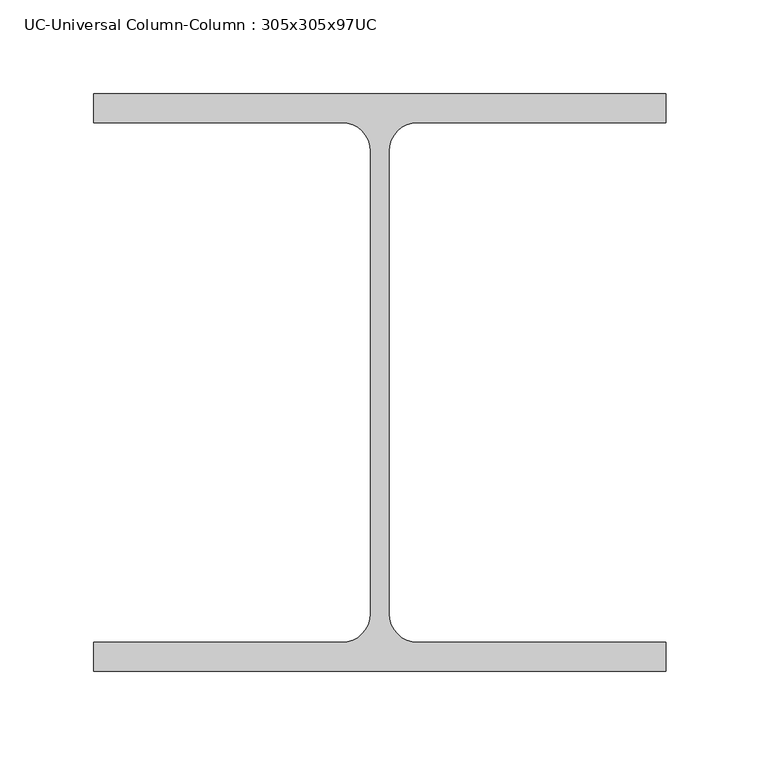
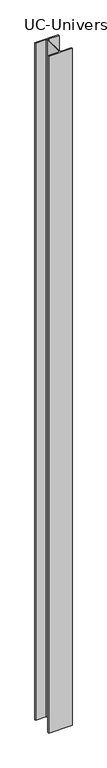
"""IFC4 building model written with IfcOpenShell, lengths in millimetres: column geometry, UC-Universal Column-Column : 305x305x97UC."""

import ifcopenshell
import ifcopenshell.guid

model = None  # the IFC model being written
_history = None  # IfcOwnerHistory: only IFC2X3 demands one
_inside = {}  # id of a spatial element -> (the spatial element, [elements in it])
_under = {}  # id of a project, library or spatial element -> (it, [spatial elements below it])
_declared = {}  # id of a project -> (the project, [libraries it declares])
_typed = {}  # id of a type object -> (the type object, [elements of that type])
_made_of = {}  # id of a material, layer set ... -> (it, [elements and type objects made of it])


def new_model(schema):
    """Start an empty IFC model of exactly this schema.

    Asked for "IFC4X3", IfcOpenShell would pick the latest addendum, in which some entities
    have other attributes; the version numbers below select the first issue.
    IFC2X3 requires an IfcOwnerHistory on every rooted entity: one is made here for all.
    """
    global model, _history
    if schema == "IFC4X3":
        model = ifcopenshell.file(schema_version=(4, 3, 0, 0))
    else:
        model = ifcopenshell.file(schema=schema)
    _inside.clear()
    _under.clear()
    _declared.clear()
    _typed.clear()
    _made_of.clear()
    _history = None
    if model.schema == "IFC2X3":
        org = make("IfcOrganization", Name="unknown")
        user = make(
            "IfcPersonAndOrganization",
            ThePerson=make("IfcPerson", FamilyName="unknown"),
            TheOrganization=org,
        )
        app = make(
            "IfcApplication",
            ApplicationDeveloper=org,
            Version="unknown",
            ApplicationFullName="unknown",
            ApplicationIdentifier="unknown",
        )
        _history = make(
            "IfcOwnerHistory",
            OwningUser=user,
            OwningApplication=app,
            ChangeAction="ADDED",
            CreationDate=0,
        )
    return model


def make(cls, **values):
    """One entity of the class cls with the attributes given. An attribute that is None is left unset."""
    return model.create_entity(
        cls, **{name: value for name, value in values.items() if value is not None}
    )


def rooted(cls, **values):
    """An entity with a GlobalId (a new one), such as an element, a storey or a relation."""
    return make(cls, GlobalId=ifcopenshell.guid.new(), OwnerHistory=_history, **values)


def si_unit(unit_type, name, prefix=None):
    """IfcSIUnit, for example si_unit("LENGTHUNIT", "METRE", prefix="MILLI")."""
    return make("IfcSIUnit", UnitType=unit_type, Prefix=prefix, Name=name)


def assignment(units):
    """IfcUnitAssignment: the units of a project."""
    return None if units is None else make("IfcUnitAssignment", Units=units)


def point(xyz):
    """IfcCartesianPoint."""
    return None if xyz is None else make("IfcCartesianPoint", Coordinates=xyz)


def direction(xyz):
    """IfcDirection."""
    return None if xyz is None else make("IfcDirection", DirectionRatios=xyz)


def frame(location, z_axis=None, x_axis=None):
    """IfcAxis2Placement3D, a coordinate frame: its origin and axes. An axis left out is left unset."""
    return make(
        "IfcAxis2Placement3D",
        Location=point(location),
        Axis=direction(z_axis),
        RefDirection=direction(x_axis),
    )


def frame_2d(location, x_axis=None):
    """IfcAxis2Placement2D, a coordinate frame in the plane: its origin and x axis."""
    return make(
        "IfcAxis2Placement2D", Location=point(location), RefDirection=direction(x_axis)
    )


def origin():
    """The frame at (0, 0, 0) with its axes left unset."""
    return frame((0.0, 0.0, 0.0))


def place(relative_to, where):
    """IfcLocalPlacement: puts the frame where relative to a parent placement (None: the world)."""
    return make(
        "IfcLocalPlacement", PlacementRelTo=relative_to, RelativePlacement=where
    )


def context(
    kind, dimensions, precision=None, world=None, true_north=None, identifier=None
):
    """IfcGeometricRepresentationContext, for example the 3D "Model" context."""
    return make(
        "IfcGeometricRepresentationContext",
        ContextIdentifier=identifier,
        ContextType=kind,
        CoordinateSpaceDimension=dimensions,
        Precision=precision,
        WorldCoordinateSystem=world,
        TrueNorth=true_north,
    )


def project(units=None, contexts=None):
    """IfcProject with its units and contexts."""
    return rooted(
        "IfcProject",
        Name="project",
        RepresentationContexts=contexts,
        UnitsInContext=assignment(units),
    )


def spatial(cls, under=None, at=None, **own):
    """A site, building, storey or space (cls), placed at a placement, below another one or the project."""
    s = rooted(cls, ObjectPlacement=at, **own)
    if under is not None:
        _under.setdefault(under.id(), (under, []))[1].append(s)
    return s


def polyline(points):
    """IfcPolyline through the points."""
    return make("IfcPolyline", Points=[point(p) for p in points])


def circle_curve(where, radius):
    """IfcCircle in the frame where."""
    return make("IfcCircle", Position=where, Radius=radius)


def trimmed(basis, trim1, trim2, sense, master):
    """IfcTrimmedCurve: the piece of a basis curve between two trims."""
    return make(
        "IfcTrimmedCurve",
        BasisCurve=basis,
        Trim1=trim1,
        Trim2=trim2,
        SenseAgreement=sense,
        MasterRepresentation=master,
    )


def segment(curve, same_sense, transition):
    """IfcCompositeCurveSegment."""
    return make(
        "IfcCompositeCurveSegment",
        Transition=transition,
        SameSense=same_sense,
        ParentCurve=curve,
    )


def composite_curve(segments, self_intersect=None):
    """IfcCompositeCurve: segments joined end to end."""
    return make("IfcCompositeCurve", Segments=segments, SelfIntersect=self_intersect)


def outline(outer, holes=None, kind="AREA"):
    """IfcArbitraryClosedProfileDef: a profile drawn as a closed curve; with holes, ...WithVoids."""
    if holes is None:
        return make("IfcArbitraryClosedProfileDef", ProfileType=kind, OuterCurve=outer)
    return make(
        "IfcArbitraryProfileDefWithVoids",
        ProfileType=kind,
        OuterCurve=outer,
        InnerCurves=holes,
    )


def extrude(swept, where, along, depth):
    """IfcExtrudedAreaSolid: the profile swept, set in the frame where, extruded along a direction by depth."""
    return make(
        "IfcExtrudedAreaSolid",
        SweptArea=swept,
        Position=where,
        ExtrudedDirection=direction(along),
        Depth=depth,
    )


def shape(context_of_items, identifier, shape_type, items):
    """IfcShapeRepresentation: the items that make up one representation, for example the "Body"."""
    return make(
        "IfcShapeRepresentation",
        ContextOfItems=context_of_items,
        RepresentationIdentifier=identifier,
        RepresentationType=shape_type,
        Items=items,
    )


def source(mapping_origin, context_of_items, identifier, shape_type, items):
    """IfcRepresentationMap: a shape defined once, which mapped items show again and again."""
    return make(
        "IfcRepresentationMap",
        MappingOrigin=mapping_origin,
        MappedRepresentation=shape(context_of_items, identifier, shape_type, items),
    )


def transform(
    local_origin,
    x_axis=None,
    y_axis=None,
    z_axis=None,
    scale=None,
    scale2=None,
    scale3=None,
    uniform=True,
):
    """IfcCartesianTransformationOperator3D, or its non-uniform kind. x_axis, y_axis, z_axis: its Axis1, 2, 3."""
    if uniform:
        return make(
            "IfcCartesianTransformationOperator3D",
            Axis1=direction(x_axis),
            Axis2=direction(y_axis),
            LocalOrigin=point(local_origin),
            Scale=scale,
            Axis3=direction(z_axis),
        )
    return make(
        "IfcCartesianTransformationOperator3DnonUniform",
        Axis1=direction(x_axis),
        Axis2=direction(y_axis),
        LocalOrigin=point(local_origin),
        Scale=scale,
        Axis3=direction(z_axis),
        Scale2=scale2,
        Scale3=scale3,
    )


def mapped(mapping_source, mapping_target):
    """IfcMappedItem: shows the shape of a source again, moved by a transform."""
    return make(
        "IfcMappedItem", MappingSource=mapping_source, MappingTarget=mapping_target
    )


def made_of(thing, what):
    """Note that an element or type object is made of a material, layer set ...; save() writes the relation."""
    if what is not None:
        _made_of.setdefault(what.id(), (what, []))[1].append(thing)
    return thing


def element(
    cls,
    number,
    at=None,
    inside=None,
    cuts=None,
    type_object=None,
    material=None,
    context=None,
    identifier="Body",
    shape_type=None,
    held_by="IfcProductDefinitionShape",
    body=None,
    shapes=None,
    **own,
):
    """One element of the class cls, such as IfcWall. Its Tag is "e" and its number.

    at: its placement. inside: the storey or other place that contains it. cuts: it is an
    opening in that element (IfcRelVoidsElement). A single representation is given by context,
    identifier, shape_type and body (its items); several are given by shapes. held_by: the class
    of the entity that holds the representations. save() writes the other relations.
    """
    e = rooted(cls, Tag="e%d" % number, ObjectPlacement=at, **own)
    if body is not None:
        shapes = [shape(context, identifier, shape_type, body)]
    if shapes is not None:
        e.Representation = make(held_by, Representations=shapes)
    if inside is not None:
        _inside.setdefault(inside.id(), (inside, []))[1].append(e)
    if cuts is not None:
        rooted(
            "IfcRelVoidsElement", RelatingBuildingElement=cuts, RelatedOpeningElement=e
        )
    if type_object is not None:
        _typed.setdefault(type_object.id(), (type_object, []))[1].append(e)
    return made_of(e, material)


def aggregate(whole, parts):
    """IfcRelAggregates: a whole, such as a stair, and the parts it consists of."""
    return rooted("IfcRelAggregates", RelatingObject=whole, RelatedObjects=parts)


def save(model, path):
    """Write the relations noted so far, then the file.

    IfcRelAggregates (storeys below a building ...), IfcRelContainedInSpatialStructure (elements
    in a storey), IfcRelDefinesByType, IfcRelAssociatesMaterial and IfcRelDeclares: one each for
    every whole, place, type object, material and project.
    """
    for whole, parts in _under.values():
        aggregate(whole, parts)
    for where, things in _inside.values():
        rooted(
            "IfcRelContainedInSpatialStructure",
            RelatedElements=things,
            RelatingStructure=where,
        )
    for kind, things in _typed.values():
        rooted("IfcRelDefinesByType", RelatedObjects=things, RelatingType=kind)
    for what, things in _made_of.values():
        rooted("IfcRelAssociatesMaterial", RelatedObjects=things, RelatingMaterial=what)
    for by, libraries in _declared.values():
        rooted("IfcRelDeclares", RelatingContext=by, RelatedDefinitions=libraries)
    model.write(path)


def uc_universal_column_column_305x305x97uc_f4bfb62a(model_context):
    return source(origin(), model_context, "Body", "SweptSolid", [
        extrude(outline(composite_curve([segment(polyline([(152.65, 153.95), (152.65, 138.55), (20.15, 138.55)]), True, "CONTINUOUS"), segment(trimmed(circle_curve(frame_2d((20.15, 123.35)), 15.2), [point((20.15, 138.55))], [point((4.95, 123.35))], True, "CARTESIAN"), True, "CONTINUOUS"), segment(polyline([(4.95, 123.35), (4.95, -123.35)]), True, "CONTINUOUS"), segment(trimmed(circle_curve(frame_2d((20.15, -123.35)), 15.2), [point((4.95, -123.35))], [point((20.15, -138.55))], True, "CARTESIAN"), True, "CONTINUOUS"), segment(polyline([(20.15, -138.55), (152.65, -138.55), (152.65, -153.95), (-152.65, -153.95), (-152.65, -138.55), (-20.15, -138.55)]), True, "CONTINUOUS"), segment(trimmed(circle_curve(frame_2d((-20.15, -123.35)), 15.2), [point((-20.15, -138.55))], [point((-4.95, -123.35))], True, "CARTESIAN"), True, "CONTINUOUS"), segment(polyline([(-4.95, -123.35), (-4.95, 123.35)]), True, "CONTINUOUS"), segment(trimmed(circle_curve(frame_2d((-20.15, 123.35)), 15.2), [point((-4.95, 123.35))], [point((-20.15, 138.55))], True, "CARTESIAN"), True, "CONTINUOUS"), segment(polyline([(-20.15, 138.55), (-152.65, 138.55), (-152.65, 153.95), (152.65, 153.95)]), True, "CONTINUOUS")], self_intersect=False)), frame((0.0, 0.0, -1500.0), z_axis=(0.0, 0.0, 1.0), x_axis=(1.0, 0.0, 0.0)), (0.0, 0.0, 1.0), 9300.0),
    ])


if __name__ == "__main__":
    model = new_model("IFC4")
    model_context = context("Model", 3, world=origin())
    ifc_project = project(units=[si_unit("LENGTHUNIT", "METRE", prefix="MILLI")], contexts=[model_context])
    site = spatial("IfcSite", under=ifc_project)
    building = spatial("IfcBuilding", under=site)
    placement = place(None, origin())
    uc_universal_column_column_305x305x97uc_shape = uc_universal_column_column_305x305x97uc_f4bfb62a(model_context)
    element("IfcColumn", 1, ObjectType="UC-Universal Column-Column : 305x305x97UC", at=placement, inside=building, context=model_context, shape_type="MappedRepresentation", body=[
        mapped(uc_universal_column_column_305x305x97uc_shape, transform((0.0, 0.0, 0.0), x_axis=(1.0, 0.0, 0.0), y_axis=(0.0, 1.0, 0.0), z_axis=(0.0, 0.0, 1.0))),
    ])
    save(model, "model.ifc")

# Revit data of these elements
# Type "UC-Universal Column-Column : 305x305x97UC"
#   Keynote = "G10"
#   Nominal h = ""
#   W = 0
#   Ix = 0
#   M = 96.9
#   Zx = 0
#   b = 305.3 mm
#   h = 307.9 mm
#   r = 15.2 mm
#   s = 9.9 mm
#   t = 15.4 mm
#   A = 123 m²
#   Structural Material [instance default] = Steel, 45-345
#   Assembly Code = ""
# Element 1 (IfcColumn, "UC-Universal Column-Column : 305x305x97UC")
#   Materials on its faces: "Steel, 45-345"
# Materials
#   "Steel, 45-345": class "Metal", colour RGB 247 247 247, transparency 0, Description = "Steel 345 MPa", Cost = 0
